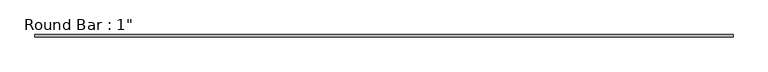
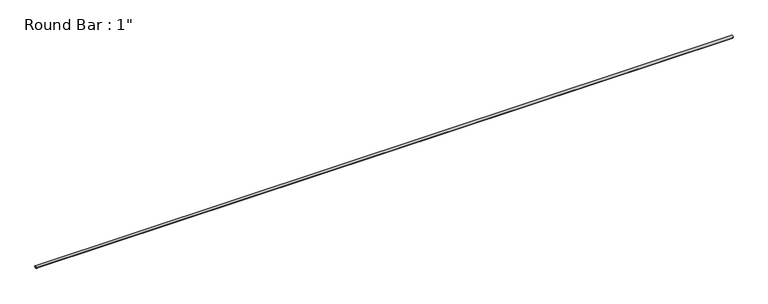
"""IFC4 building model written with IfcOpenShell, lengths in millimetres: member geometry."""

import ifcopenshell
import ifcopenshell.guid

model = None  # the IFC model being written
_history = None  # IfcOwnerHistory: only IFC2X3 demands one
_inside = {}  # id of a spatial element -> (the spatial element, [elements in it])
_under = {}  # id of a project, library or spatial element -> (it, [spatial elements below it])
_declared = {}  # id of a project -> (the project, [libraries it declares])
_typed = {}  # id of a type object -> (the type object, [elements of that type])
_made_of = {}  # id of a material, layer set ... -> (it, [elements and type objects made of it])


def new_model(schema):
    """Start an empty IFC model of exactly this schema.

    Asked for "IFC4X3", IfcOpenShell would pick the latest addendum, in which some entities
    have other attributes; the version numbers below select the first issue.
    IFC2X3 requires an IfcOwnerHistory on every rooted entity: one is made here for all.
    """
    global model, _history
    if schema == "IFC4X3":
        model = ifcopenshell.file(schema_version=(4, 3, 0, 0))
    else:
        model = ifcopenshell.file(schema=schema)
    _inside.clear()
    _under.clear()
    _declared.clear()
    _typed.clear()
    _made_of.clear()
    _history = None
    if model.schema == "IFC2X3":
        org = make("IfcOrganization", Name="unknown")
        user = make(
            "IfcPersonAndOrganization",
            ThePerson=make("IfcPerson", FamilyName="unknown"),
            TheOrganization=org,
        )
        app = make(
            "IfcApplication",
            ApplicationDeveloper=org,
            Version="unknown",
            ApplicationFullName="unknown",
            ApplicationIdentifier="unknown",
        )
        _history = make(
            "IfcOwnerHistory",
            OwningUser=user,
            OwningApplication=app,
            ChangeAction="ADDED",
            CreationDate=0,
        )
    return model


def make(cls, **values):
    """One entity of the class cls with the attributes given. An attribute that is None is left unset."""
    return model.create_entity(
        cls, **{name: value for name, value in values.items() if value is not None}
    )


def rooted(cls, **values):
    """An entity with a GlobalId (a new one), such as an element, a storey or a relation."""
    return make(cls, GlobalId=ifcopenshell.guid.new(), OwnerHistory=_history, **values)


def si_unit(unit_type, name, prefix=None):
    """IfcSIUnit, for example si_unit("LENGTHUNIT", "METRE", prefix="MILLI")."""
    return make("IfcSIUnit", UnitType=unit_type, Prefix=prefix, Name=name)


def assignment(units):
    """IfcUnitAssignment: the units of a project."""
    return None if units is None else make("IfcUnitAssignment", Units=units)


def point(xyz):
    """IfcCartesianPoint."""
    return None if xyz is None else make("IfcCartesianPoint", Coordinates=xyz)


def direction(xyz):
    """IfcDirection."""
    return None if xyz is None else make("IfcDirection", DirectionRatios=xyz)


def frame(location, z_axis=None, x_axis=None):
    """IfcAxis2Placement3D, a coordinate frame: its origin and axes. An axis left out is left unset."""
    return make(
        "IfcAxis2Placement3D",
        Location=point(location),
        Axis=direction(z_axis),
        RefDirection=direction(x_axis),
    )


def frame_2d(location, x_axis=None):
    """IfcAxis2Placement2D, a coordinate frame in the plane: its origin and x axis."""
    return make(
        "IfcAxis2Placement2D", Location=point(location), RefDirection=direction(x_axis)
    )


def origin():
    """The frame at (0, 0, 0) with its axes left unset."""
    return frame((0.0, 0.0, 0.0))


def origin_2d():
    """The frame at (0, 0) in the plane with its x axis left unset."""
    return frame_2d((0.0, 0.0))


def place(relative_to, where):
    """IfcLocalPlacement: puts the frame where relative to a parent placement (None: the world)."""
    return make(
        "IfcLocalPlacement", PlacementRelTo=relative_to, RelativePlacement=where
    )


def context(
    kind, dimensions, precision=None, world=None, true_north=None, identifier=None
):
    """IfcGeometricRepresentationContext, for example the 3D "Model" context."""
    return make(
        "IfcGeometricRepresentationContext",
        ContextIdentifier=identifier,
        ContextType=kind,
        CoordinateSpaceDimension=dimensions,
        Precision=precision,
        WorldCoordinateSystem=world,
        TrueNorth=true_north,
    )


def project(units=None, contexts=None):
    """IfcProject with its units and contexts."""
    return rooted(
        "IfcProject",
        Name="project",
        RepresentationContexts=contexts,
        UnitsInContext=assignment(units),
    )


def spatial(cls, under=None, at=None, **own):
    """A site, building, storey or space (cls), placed at a placement, below another one or the project."""
    s = rooted(cls, ObjectPlacement=at, **own)
    if under is not None:
        _under.setdefault(under.id(), (under, []))[1].append(s)
    return s


def circle_curve(where, radius):
    """IfcCircle in the frame where."""
    return make("IfcCircle", Position=where, Radius=radius)


def trimmed(basis, trim1, trim2, sense, master):
    """IfcTrimmedCurve: the piece of a basis curve between two trims."""
    return make(
        "IfcTrimmedCurve",
        BasisCurve=basis,
        Trim1=trim1,
        Trim2=trim2,
        SenseAgreement=sense,
        MasterRepresentation=master,
    )


def segment(curve, same_sense, transition):
    """IfcCompositeCurveSegment."""
    return make(
        "IfcCompositeCurveSegment",
        Transition=transition,
        SameSense=same_sense,
        ParentCurve=curve,
    )


def composite_curve(segments, self_intersect=None):
    """IfcCompositeCurve: segments joined end to end."""
    return make("IfcCompositeCurve", Segments=segments, SelfIntersect=self_intersect)


def outline(outer, holes=None, kind="AREA"):
    """IfcArbitraryClosedProfileDef: a profile drawn as a closed curve; with holes, ...WithVoids."""
    if holes is None:
        return make("IfcArbitraryClosedProfileDef", ProfileType=kind, OuterCurve=outer)
    return make(
        "IfcArbitraryProfileDefWithVoids",
        ProfileType=kind,
        OuterCurve=outer,
        InnerCurves=holes,
    )


def extrude(swept, where, along, depth):
    """IfcExtrudedAreaSolid: the profile swept, set in the frame where, extruded along a direction by depth."""
    return make(
        "IfcExtrudedAreaSolid",
        SweptArea=swept,
        Position=where,
        ExtrudedDirection=direction(along),
        Depth=depth,
    )


def shape(context_of_items, identifier, shape_type, items):
    """IfcShapeRepresentation: the items that make up one representation, for example the "Body"."""
    return make(
        "IfcShapeRepresentation",
        ContextOfItems=context_of_items,
        RepresentationIdentifier=identifier,
        RepresentationType=shape_type,
        Items=items,
    )


def source(mapping_origin, context_of_items, identifier, shape_type, items):
    """IfcRepresentationMap: a shape defined once, which mapped items show again and again."""
    return make(
        "IfcRepresentationMap",
        MappingOrigin=mapping_origin,
        MappedRepresentation=shape(context_of_items, identifier, shape_type, items),
    )


def transform(
    local_origin,
    x_axis=None,
    y_axis=None,
    z_axis=None,
    scale=None,
    scale2=None,
    scale3=None,
    uniform=True,
):
    """IfcCartesianTransformationOperator3D, or its non-uniform kind. x_axis, y_axis, z_axis: its Axis1, 2, 3."""
    if uniform:
        return make(
            "IfcCartesianTransformationOperator3D",
            Axis1=direction(x_axis),
            Axis2=direction(y_axis),
            LocalOrigin=point(local_origin),
            Scale=scale,
            Axis3=direction(z_axis),
        )
    return make(
        "IfcCartesianTransformationOperator3DnonUniform",
        Axis1=direction(x_axis),
        Axis2=direction(y_axis),
        LocalOrigin=point(local_origin),
        Scale=scale,
        Axis3=direction(z_axis),
        Scale2=scale2,
        Scale3=scale3,
    )


def mapped(mapping_source, mapping_target):
    """IfcMappedItem: shows the shape of a source again, moved by a transform."""
    return make(
        "IfcMappedItem", MappingSource=mapping_source, MappingTarget=mapping_target
    )


def made_of(thing, what):
    """Note that an element or type object is made of a material, layer set ...; save() writes the relation."""
    if what is not None:
        _made_of.setdefault(what.id(), (what, []))[1].append(thing)
    return thing


def element(
    cls,
    number,
    at=None,
    inside=None,
    cuts=None,
    type_object=None,
    material=None,
    context=None,
    identifier="Body",
    shape_type=None,
    held_by="IfcProductDefinitionShape",
    body=None,
    shapes=None,
    **own,
):
    """One element of the class cls, such as IfcWall. Its Tag is "e" and its number.

    at: its placement. inside: the storey or other place that contains it. cuts: it is an
    opening in that element (IfcRelVoidsElement). A single representation is given by context,
    identifier, shape_type and body (its items); several are given by shapes. held_by: the class
    of the entity that holds the representations. save() writes the other relations.
    """
    e = rooted(cls, Tag="e%d" % number, ObjectPlacement=at, **own)
    if body is not None:
        shapes = [shape(context, identifier, shape_type, body)]
    if shapes is not None:
        e.Representation = make(held_by, Representations=shapes)
    if inside is not None:
        _inside.setdefault(inside.id(), (inside, []))[1].append(e)
    if cuts is not None:
        rooted(
            "IfcRelVoidsElement", RelatingBuildingElement=cuts, RelatedOpeningElement=e
        )
    if type_object is not None:
        _typed.setdefault(type_object.id(), (type_object, []))[1].append(e)
    return made_of(e, material)


def aggregate(whole, parts):
    """IfcRelAggregates: a whole, such as a stair, and the parts it consists of."""
    return rooted("IfcRelAggregates", RelatingObject=whole, RelatedObjects=parts)


def save(model, path):
    """Write the relations noted so far, then the file.

    IfcRelAggregates (storeys below a building ...), IfcRelContainedInSpatialStructure (elements
    in a storey), IfcRelDefinesByType, IfcRelAssociatesMaterial and IfcRelDeclares: one each for
    every whole, place, type object, material and project.
    """
    for whole, parts in _under.values():
        aggregate(whole, parts)
    for where, things in _inside.values():
        rooted(
            "IfcRelContainedInSpatialStructure",
            RelatedElements=things,
            RelatingStructure=where,
        )
    for kind, things in _typed.values():
        rooted("IfcRelDefinesByType", RelatedObjects=things, RelatingType=kind)
    for what, things in _made_of.values():
        rooted("IfcRelAssociatesMaterial", RelatedObjects=things, RelatingMaterial=what)
    for by, libraries in _declared.values():
        rooted("IfcRelDeclares", RelatingContext=by, RelatedDefinitions=libraries)
    model.write(path)


def member_357c6e14(model_context):
    return source(origin(), model_context, "Body", "SweptSolid", [
        extrude(outline(composite_curve([segment(trimmed(circle_curve(origin_2d(), 12.7), [point((12.7, 0.0))], [point((-12.7, 0.0))], False, "CARTESIAN"), True, "CONTINUOUS"), segment(trimmed(circle_curve(origin_2d(), 12.7), [point((-12.7, 0.0))], [point((12.7, 0.0))], False, "CARTESIAN"), True, "CONTINUOUS")], self_intersect=False)), frame((-3554.2056387, 0.0, 0.0), z_axis=(1.0, 0.0, 0.0), x_axis=(0.0, 1.0, 0.0)), (0.0, 0.0, 1.0), 7108.4112774),
    ])


if __name__ == "__main__":
    model = new_model("IFC4")
    model_context = context("Model", 3, world=origin())
    ifc_project = project(units=[si_unit("LENGTHUNIT", "METRE", prefix="MILLI")], contexts=[model_context])
    site = spatial("IfcSite", under=ifc_project)
    building = spatial("IfcBuilding", under=site)
    placement = place(None, origin())
    member_shape = member_357c6e14(model_context)
    element("IfcMember", 1, ObjectType="Round Bar : 1\"", at=placement, inside=building, context=model_context, shape_type="MappedRepresentation", body=[
        mapped(member_shape, transform((0.0, 0.0, 0.0), x_axis=(1.0, 0.0, 0.0), y_axis=(0.0, 1.0, 0.0), z_axis=(0.0, 0.0, 1.0))),
    ])
    save(model, "model.ifc")

# Revit data of these elements
# Type "Round Bar : 1\""
#   Assembly Code = "B10"
#   W = 0
#   Start Extension Calculation [instance default] = 10' - 0"
#   Start Extension [instance default] = -0' - 0 1/2"
#   End Extension Calculation [instance default] = 10' - 0"
#   End Extension [instance default] = -0' - 0 1/2"
#   Length [instance default] = 5' - 0"
#   d = 0' - 1"
#   A = 0 SF
#   Structural Material [instance default] = Metal - Steel - ASTM A36
# Element 1 (IfcMember, "Round Bar : 1\"")
#   Materials on its faces: "Metal - Steel - ASTM A36"
# Materials
#   "Metal - Steel - ASTM A36": class "Metal", colour RGB 199 199 199, transparency 0
